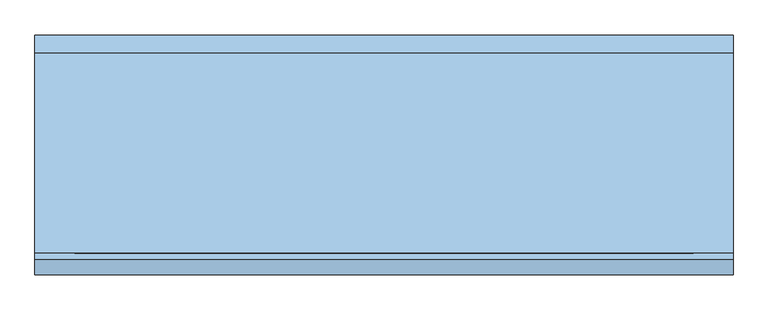
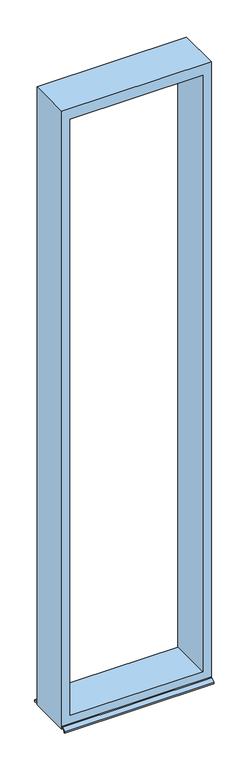
"""IFC4 building model written with IfcOpenShell, lengths in millimetres: window geometry, Fenster - Festverglasung : Feste Verglasung 4.58 x 1.05 2."""

from ifc_helpers import new_model, si_unit, frame, origin, place, context, project, spatial, polyline, outline, extrude, source, transform, mapped, element, save


def window_c1246823(model_context):
    return source(origin(), model_context, "Body", "SweptSolid", [
        extrude(outline(polyline([(5580.0, 525.0), (5580.0, -525.0), (1000.0, -525.0), (1000.0, 525.0), (5580.0, 525.0)]), holes=[polyline([(5500.0, 465.0), (1080.0, 465.0), (1080.0, -465.0), (5500.0, -465.0), (5500.0, 465.0)])]), frame((0.0, -147.5214598, 0.0), z_axis=(0.0, 1.0, 0.0), x_axis=(0.0, 0.0, 1.0)), (0.0, 0.0, 1.0), 300.0),
        extrude(outline(polyline([(-525.0, 180.0), (525.0, 180.0), (525.0, 152.4785402), (-525.0, 152.4785402), (-525.0, 180.0)])), frame((0.0, 0.0, 1005.0), z_axis=(0.0, 0.0, 1.0), x_axis=(1.0, 0.0, 0.0)), (0.0, 0.0, 1.0), 15.0),
        extrude(outline(polyline([(-157.5436142, 1020.0), (-147.5214598, 1020.0), (-147.5214598, 1018.0), (-157.3455321, 1018.0), (-178.0, 998.3604634), (-178.0, 990.0), (-180.0, 990.0), (-180.0, 1000.0), (-157.5436142, 1020.0)])), frame((-525.0, 0.0, 0.0), z_axis=(1.0, 0.0, 0.0), x_axis=(0.0, 1.0, 0.0)), (0.0, 0.0, 1.0), 1050.0),
    ])


if __name__ == "__main__":
    model = new_model("IFC4")
    model_context = context("Model", 3, world=origin())
    ifc_project = project(units=[si_unit("LENGTHUNIT", "METRE", prefix="MILLI")], contexts=[model_context])
    site = spatial("IfcSite", under=ifc_project)
    building = spatial("IfcBuilding", under=site)
    placement = place(None, origin())
    window_shape = window_c1246823(model_context)
    element("IfcWindow", 1, ObjectType="Fenster - Festverglasung : Feste Verglasung 4.58 x 1.05 2", at=placement, inside=building, context=model_context, shape_type="MappedRepresentation", body=[
        mapped(window_shape, transform((0.0, 0.0, 0.0), x_axis=(1.0, 0.0, 0.0), y_axis=(0.0, 1.0, 0.0), z_axis=(0.0, 0.0, 1.0))),
    ])
    save(model, "model.ifc")

# Revit data of these elements
# Type "Fenster - Festverglasung : Feste Verglasung 4.58 x 1.05 2"
#   Type Mark = "69"
#   Operation = "SinglePanel"
#   Keynote = "16.05.01"
#   Visual Light Transmittance = 0.9
#   Solar Heat Gain Coefficient = 0.78
#   Rough Width = 1.050 m
#   Rough Height = 4.580 m
#   Heat Transfer Coefficient (U) = 3.6886 W/(m²·K)
#   Rahmentiefe = 0.300 m
#   Rahmenhöhe unten = 0.080 m
#   Höhe oberer  Rahmen = 0.080 m
#   Rahmenbreite = 0.060 m
#   Height = 4.580 m
#   Einbautiefe (von außen) [instance default] = 0.080 m
#   Width = 1.050 m
#   Wall Closure = 3
#   Bild [instance default] = none
#   Glas [instance default] = none
#   Innere Fensterbank [instance default] = none
#   Äußere Fensterbank [instance default] = none
#   Construction Type Id = ""
#   Analytic Construction = (empty or 0)
# Element 1 (IfcWindow, "Fenster - Festverglasung : Feste Verglasung 4.58 x 1.05 2")
#   Einbautiefe (von außen) = 0.002479 m
#   Materials on its faces: "Kunststoff - Weiß", "Holz - Birke"
# Materials
#   "Kunststoff - Weiß": class "Kunststoff", colour RGB 249 249 249, transparency 0, Cost = 0
#   "Holz - Birke": class "Holz", colour RGB 213 164 103, transparency 0, Cost = 0
